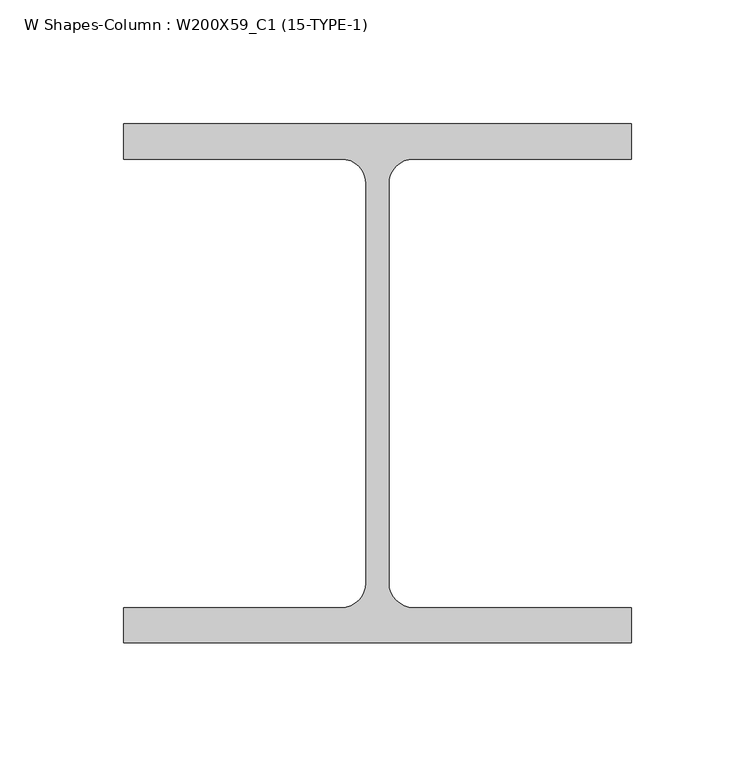
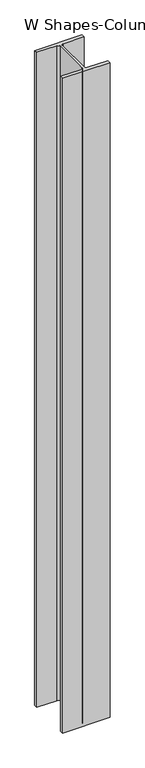
"""IFC4 building model written with IfcOpenShell, lengths in millimetres: column geometry, W Shapes-Column : W200X59_C1 (15-TYPE-1)."""

from ifc_helpers import new_model, si_unit, point, frame, frame_2d, origin, place, context, project, spatial, polyline, circle_curve, trimmed, segment, composite_curve, outline, extrude, source, transform, mapped, element, save


def w_shapes_column_w200x59_c1_15_type_1_c42af12d(model_context):
    return source(origin(), model_context, "Body", "SweptSolid", [
        extrude(outline(composite_curve([segment(polyline([(102.489, 104.775), (102.489, 90.551), (14.5796, 90.551)]), True, "CONTINUOUS"), segment(trimmed(circle_curve(frame_2d((14.5796, 80.5434)), 10.0076), [point((14.5796, 90.551))], [point((4.572, 80.5434))], True, "CARTESIAN"), True, "CONTINUOUS"), segment(polyline([(4.572, 80.5434), (4.572, -80.5434)]), True, "CONTINUOUS"), segment(trimmed(circle_curve(frame_2d((14.5796, -80.5434)), 10.0076), [point((4.572, -80.5434))], [point((14.5796, -90.551))], True, "CARTESIAN"), True, "CONTINUOUS"), segment(polyline([(14.5796, -90.551), (102.489, -90.551), (102.489, -104.775), (-102.489, -104.775), (-102.489, -90.551), (-14.5796, -90.551)]), True, "CONTINUOUS"), segment(trimmed(circle_curve(frame_2d((-14.5796, -80.5434)), 10.0076), [point((-14.5796, -90.551))], [point((-4.572, -80.5434))], True, "CARTESIAN"), True, "CONTINUOUS"), segment(polyline([(-4.572, -80.5434), (-4.572, 80.5434)]), True, "CONTINUOUS"), segment(trimmed(circle_curve(frame_2d((-14.5796, 80.5434)), 10.0076), [point((-4.572, 80.5434))], [point((-14.5796, 90.551))], True, "CARTESIAN"), True, "CONTINUOUS"), segment(polyline([(-14.5796, 90.551), (-102.489, 90.551), (-102.489, 104.775), (102.489, 104.775)]), True, "CONTINUOUS")], self_intersect=False)), frame((0.0, 0.0, 200.0), z_axis=(0.0, 0.0, 1.0), x_axis=(1.0, 0.0, 0.0)), (0.0, 0.0, 1.0), 3000.0),
    ])


if __name__ == "__main__":
    model = new_model("IFC4")
    model_context = context("Model", 3, world=origin())
    ifc_project = project(units=[si_unit("LENGTHUNIT", "METRE", prefix="MILLI")], contexts=[model_context])
    site = spatial("IfcSite", under=ifc_project)
    building = spatial("IfcBuilding", under=site)
    placement = place(None, origin())
    w_shapes_column_w200x59_c1_15_type_1_shape = w_shapes_column_w200x59_c1_15_type_1_c42af12d(model_context)
    element("IfcColumn", 1, ObjectType="W Shapes-Column : W200X59_C1 (15-TYPE-1)", at=placement, inside=building, context=model_context, shape_type="MappedRepresentation", body=[
        mapped(w_shapes_column_w200x59_c1_15_type_1_shape, transform((0.0, 0.0, 0.0), x_axis=(1.0, 0.0, 0.0), y_axis=(0.0, 1.0, 0.0), z_axis=(0.0, 0.0, 1.0))),
    ])
    save(model, "model.ifc")

# Revit data of these elements
# Type "W Shapes-Column : W200X59_C1 (15-TYPE-1)"
#   Section Name Key = "W8x40"
#   Assembly Code = "B10"
#   Width = 20.4978 cm
#   Web Thickness = 0.9144 cm
#   Web Fillet = 1.0008 cm
#   Warping Constant = 194957.0 cm⁶
#   Torsional Moment of Inertia = 46.6179 cm⁴
#   Section Area = 75.4837 cm²
#   Plastic Modulus weak axis = 303.161 cm³
#   Plastic Modulus strong axis = 652.205 cm³
#   Perimeter = 1.20396 m²/m
#   Nominal Weight = 59.5266 kgf/m
#   Moment of Inertia weak axis = 2043.70 cm⁴
#   Moment of Inertia strong axis = 6076.98 cm⁴
#   Height = 20.955 cm
#   Flange Thickness = 1.4224 cm
#   Elastic Modulus weak axis = 199.922 cm³
#   Elastic Modulus strong axis = 581.741 cm³
#   Clear Web Height = 19.05 cm
#   Centroid Vertical = 10.4775 cm
#   Centroid Horizontal = 10.2489 cm
#   Bolt Spacing = 13.97 cm
#   Structural Material [instance default] = Steel ASTM A992
#   Principal Axes Angle = 0
# Element 1 (IfcColumn, "W Shapes-Column : W200X59_C1 (15-TYPE-1)")
#   Structural Material = none
# Materials
#   "Steel ASTM A992": class "Metal", colour RGB 199 199 199, transparency 0, Description = "Structural steel 50ksi", Cost = 0
